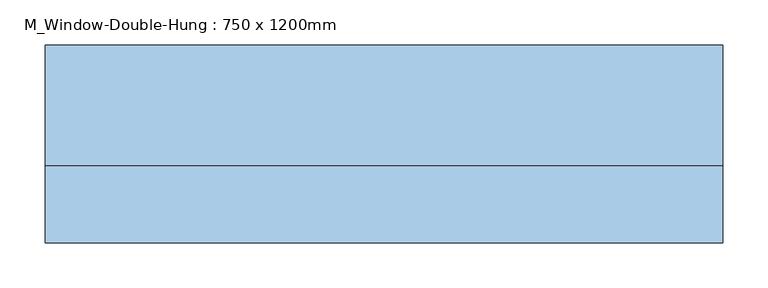
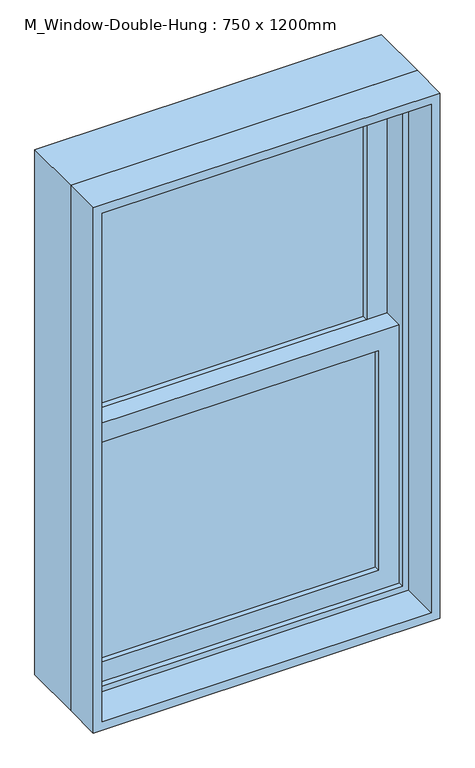
"""IFC4 building model written with IfcOpenShell, lengths in millimetres: window geometry, M_Window-Double-Hung : 750 x 1200mm."""

import ifcopenshell
import ifcopenshell.guid

model = None  # the IFC model being written
_history = None  # IfcOwnerHistory: only IFC2X3 demands one
_inside = {}  # id of a spatial element -> (the spatial element, [elements in it])
_under = {}  # id of a project, library or spatial element -> (it, [spatial elements below it])
_declared = {}  # id of a project -> (the project, [libraries it declares])
_typed = {}  # id of a type object -> (the type object, [elements of that type])
_made_of = {}  # id of a material, layer set ... -> (it, [elements and type objects made of it])


def new_model(schema):
    """Start an empty IFC model of exactly this schema.

    Asked for "IFC4X3", IfcOpenShell would pick the latest addendum, in which some entities
    have other attributes; the version numbers below select the first issue.
    IFC2X3 requires an IfcOwnerHistory on every rooted entity: one is made here for all.
    """
    global model, _history
    if schema == "IFC4X3":
        model = ifcopenshell.file(schema_version=(4, 3, 0, 0))
    else:
        model = ifcopenshell.file(schema=schema)
    _inside.clear()
    _under.clear()
    _declared.clear()
    _typed.clear()
    _made_of.clear()
    _history = None
    if model.schema == "IFC2X3":
        org = make("IfcOrganization", Name="unknown")
        user = make(
            "IfcPersonAndOrganization",
            ThePerson=make("IfcPerson", FamilyName="unknown"),
            TheOrganization=org,
        )
        app = make(
            "IfcApplication",
            ApplicationDeveloper=org,
            Version="unknown",
            ApplicationFullName="unknown",
            ApplicationIdentifier="unknown",
        )
        _history = make(
            "IfcOwnerHistory",
            OwningUser=user,
            OwningApplication=app,
            ChangeAction="ADDED",
            CreationDate=0,
        )
    return model


def make(cls, **values):
    """One entity of the class cls with the attributes given. An attribute that is None is left unset."""
    return model.create_entity(
        cls, **{name: value for name, value in values.items() if value is not None}
    )


def rooted(cls, **values):
    """An entity with a GlobalId (a new one), such as an element, a storey or a relation."""
    return make(cls, GlobalId=ifcopenshell.guid.new(), OwnerHistory=_history, **values)


def si_unit(unit_type, name, prefix=None):
    """IfcSIUnit, for example si_unit("LENGTHUNIT", "METRE", prefix="MILLI")."""
    return make("IfcSIUnit", UnitType=unit_type, Prefix=prefix, Name=name)


def assignment(units):
    """IfcUnitAssignment: the units of a project."""
    return None if units is None else make("IfcUnitAssignment", Units=units)


def point(xyz):
    """IfcCartesianPoint."""
    return None if xyz is None else make("IfcCartesianPoint", Coordinates=xyz)


def direction(xyz):
    """IfcDirection."""
    return None if xyz is None else make("IfcDirection", DirectionRatios=xyz)


def frame(location, z_axis=None, x_axis=None):
    """IfcAxis2Placement3D, a coordinate frame: its origin and axes. An axis left out is left unset."""
    return make(
        "IfcAxis2Placement3D",
        Location=point(location),
        Axis=direction(z_axis),
        RefDirection=direction(x_axis),
    )


def origin():
    """The frame at (0, 0, 0) with its axes left unset."""
    return frame((0.0, 0.0, 0.0))


def place(relative_to, where):
    """IfcLocalPlacement: puts the frame where relative to a parent placement (None: the world)."""
    return make(
        "IfcLocalPlacement", PlacementRelTo=relative_to, RelativePlacement=where
    )


def context(
    kind, dimensions, precision=None, world=None, true_north=None, identifier=None
):
    """IfcGeometricRepresentationContext, for example the 3D "Model" context."""
    return make(
        "IfcGeometricRepresentationContext",
        ContextIdentifier=identifier,
        ContextType=kind,
        CoordinateSpaceDimension=dimensions,
        Precision=precision,
        WorldCoordinateSystem=world,
        TrueNorth=true_north,
    )


def project(units=None, contexts=None):
    """IfcProject with its units and contexts."""
    return rooted(
        "IfcProject",
        Name="project",
        RepresentationContexts=contexts,
        UnitsInContext=assignment(units),
    )


def spatial(cls, under=None, at=None, **own):
    """A site, building, storey or space (cls), placed at a placement, below another one or the project."""
    s = rooted(cls, ObjectPlacement=at, **own)
    if under is not None:
        _under.setdefault(under.id(), (under, []))[1].append(s)
    return s


def polyline(points):
    """IfcPolyline through the points."""
    return make("IfcPolyline", Points=[point(p) for p in points])


def outline(outer, holes=None, kind="AREA"):
    """IfcArbitraryClosedProfileDef: a profile drawn as a closed curve; with holes, ...WithVoids."""
    if holes is None:
        return make("IfcArbitraryClosedProfileDef", ProfileType=kind, OuterCurve=outer)
    return make(
        "IfcArbitraryProfileDefWithVoids",
        ProfileType=kind,
        OuterCurve=outer,
        InnerCurves=holes,
    )


def extrude(swept, where, along, depth):
    """IfcExtrudedAreaSolid: the profile swept, set in the frame where, extruded along a direction by depth."""
    return make(
        "IfcExtrudedAreaSolid",
        SweptArea=swept,
        Position=where,
        ExtrudedDirection=direction(along),
        Depth=depth,
    )


def shape(context_of_items, identifier, shape_type, items):
    """IfcShapeRepresentation: the items that make up one representation, for example the "Body"."""
    return make(
        "IfcShapeRepresentation",
        ContextOfItems=context_of_items,
        RepresentationIdentifier=identifier,
        RepresentationType=shape_type,
        Items=items,
    )


def source(mapping_origin, context_of_items, identifier, shape_type, items):
    """IfcRepresentationMap: a shape defined once, which mapped items show again and again."""
    return make(
        "IfcRepresentationMap",
        MappingOrigin=mapping_origin,
        MappedRepresentation=shape(context_of_items, identifier, shape_type, items),
    )


def transform(
    local_origin,
    x_axis=None,
    y_axis=None,
    z_axis=None,
    scale=None,
    scale2=None,
    scale3=None,
    uniform=True,
):
    """IfcCartesianTransformationOperator3D, or its non-uniform kind. x_axis, y_axis, z_axis: its Axis1, 2, 3."""
    if uniform:
        return make(
            "IfcCartesianTransformationOperator3D",
            Axis1=direction(x_axis),
            Axis2=direction(y_axis),
            LocalOrigin=point(local_origin),
            Scale=scale,
            Axis3=direction(z_axis),
        )
    return make(
        "IfcCartesianTransformationOperator3DnonUniform",
        Axis1=direction(x_axis),
        Axis2=direction(y_axis),
        LocalOrigin=point(local_origin),
        Scale=scale,
        Axis3=direction(z_axis),
        Scale2=scale2,
        Scale3=scale3,
    )


def mapped(mapping_source, mapping_target):
    """IfcMappedItem: shows the shape of a source again, moved by a transform."""
    return make(
        "IfcMappedItem", MappingSource=mapping_source, MappingTarget=mapping_target
    )


def made_of(thing, what):
    """Note that an element or type object is made of a material, layer set ...; save() writes the relation."""
    if what is not None:
        _made_of.setdefault(what.id(), (what, []))[1].append(thing)
    return thing


def element(
    cls,
    number,
    at=None,
    inside=None,
    cuts=None,
    type_object=None,
    material=None,
    context=None,
    identifier="Body",
    shape_type=None,
    held_by="IfcProductDefinitionShape",
    body=None,
    shapes=None,
    **own,
):
    """One element of the class cls, such as IfcWall. Its Tag is "e" and its number.

    at: its placement. inside: the storey or other place that contains it. cuts: it is an
    opening in that element (IfcRelVoidsElement). A single representation is given by context,
    identifier, shape_type and body (its items); several are given by shapes. held_by: the class
    of the entity that holds the representations. save() writes the other relations.
    """
    e = rooted(cls, Tag="e%d" % number, ObjectPlacement=at, **own)
    if body is not None:
        shapes = [shape(context, identifier, shape_type, body)]
    if shapes is not None:
        e.Representation = make(held_by, Representations=shapes)
    if inside is not None:
        _inside.setdefault(inside.id(), (inside, []))[1].append(e)
    if cuts is not None:
        rooted(
            "IfcRelVoidsElement", RelatingBuildingElement=cuts, RelatedOpeningElement=e
        )
    if type_object is not None:
        _typed.setdefault(type_object.id(), (type_object, []))[1].append(e)
    return made_of(e, material)


def aggregate(whole, parts):
    """IfcRelAggregates: a whole, such as a stair, and the parts it consists of."""
    return rooted("IfcRelAggregates", RelatingObject=whole, RelatedObjects=parts)


def save(model, path):
    """Write the relations noted so far, then the file.

    IfcRelAggregates (storeys below a building ...), IfcRelContainedInSpatialStructure (elements
    in a storey), IfcRelDefinesByType, IfcRelAssociatesMaterial and IfcRelDeclares: one each for
    every whole, place, type object, material and project.
    """
    for whole, parts in _under.values():
        aggregate(whole, parts)
    for where, things in _inside.values():
        rooted(
            "IfcRelContainedInSpatialStructure",
            RelatedElements=things,
            RelatingStructure=where,
        )
    for kind, things in _typed.values():
        rooted("IfcRelDefinesByType", RelatedObjects=things, RelatingType=kind)
    for what, things in _made_of.values():
        rooted("IfcRelAssociatesMaterial", RelatedObjects=things, RelatingMaterial=what)
    for by, libraries in _declared.values():
        rooted("IfcRelDeclares", RelatingContext=by, RelatedDefinitions=libraries)
    model.write(path)


def m_window_double_hung_750_x_1200mm_41070976(model_context):
    return source(origin(), model_context, "Body", "SweptSolid", [
        extrude(outline(polyline([(298.8, 30.15), (298.8, 23.8), (-298.8, 23.8), (-298.8, 30.15), (298.8, 30.15)])), frame((0.0, 0.0, 990.6), z_axis=(0.0, 0.0, 1.0), x_axis=(1.0, 0.0, 0.0)), (0.0, 0.0, 1.0), 501.575),
        extrude(outline(polyline([(-298.8, 17.45), (298.8, 17.45), (298.8, 11.1), (-298.8, 11.1), (-298.8, 17.45)])), frame((0.0, 0.0, 990.6), z_axis=(0.0, 0.0, 1.0), x_axis=(1.0, 0.0, 0.0)), (0.0, 0.0, 1.0), 501.575),
        extrude(outline(polyline([(298.8, 74.6), (298.8, 68.25), (-298.8, 68.25), (-298.8, 74.6), (298.8, 74.6)])), frame((0.0, 0.0, 1536.625), z_axis=(0.0, 0.0, 1.0), x_axis=(1.0, 0.0, 0.0)), (0.0, 0.0, 1.0), 501.575),
        extrude(outline(polyline([(-298.8, 61.9), (298.8, 61.9), (298.8, 55.55), (-298.8, 55.55), (-298.8, 61.9)])), frame((0.0, 0.0, 1536.625), z_axis=(0.0, 0.0, 1.0), x_axis=(1.0, 0.0, 0.0)), (0.0, 0.0, 1.0), 501.575),
        extrude(outline(polyline([(1536.625, -343.25), (946.15, -343.25), (946.15, 343.25), (1536.625, 343.25), (1536.625, -343.25)]), holes=[polyline([(1492.175, 298.8), (990.6, 298.8), (990.6, -298.8), (1492.175, -298.8), (1492.175, 298.8)])]), frame((0.0, -1.6, 0.0), z_axis=(0.0, 1.0, 0.0), x_axis=(0.0, 0.0, 1.0)), (0.0, 0.0, 1.0), 44.45),
        extrude(outline(polyline([(2082.65, -343.25), (1492.175, -343.25), (1492.175, 343.25), (2082.65, 343.25), (2082.65, -343.25)]), holes=[polyline([(2038.2, 298.8), (1536.625, 298.8), (1536.625, -298.8), (2038.2, -298.8), (2038.2, 298.8)])]), frame((0.0, 42.85, 0.0), z_axis=(0.0, 1.0, 0.0), x_axis=(0.0, 0.0, 1.0)), (0.0, 0.0, 1.0), 44.45),
        extrude(outline(polyline([(2114.4, -375.0), (914.4, -375.0), (914.4, 375.0), (2114.4, 375.0), (2114.4, -375.0)]), holes=[polyline([(2082.65, 343.25), (946.15, 343.25), (946.15, -343.25), (2082.65, -343.25), (2082.65, 343.25)])]), frame((0.0, -14.3, 0.0), z_axis=(0.0, 1.0, 0.0), x_axis=(0.0, 0.0, 1.0)), (0.0, 0.0, 1.0), 133.35),
        extrude(outline(polyline([(2114.4, 375.0), (2114.4, -375.0), (914.4, -375.0), (914.4, 375.0), (2114.4, 375.0)]), holes=[polyline([(2095.35, 355.95), (933.45, 355.95), (933.45, -355.95), (2095.35, -355.95), (2095.35, 355.95)])]), frame((0.0, -100.0, 0.0), z_axis=(0.0, 1.0, 0.0), x_axis=(0.0, 0.0, 1.0)), (0.0, 0.0, 1.0), 85.7),
    ])


if __name__ == "__main__":
    model = new_model("IFC4")
    model_context = context("Model", 3, world=origin())
    ifc_project = project(units=[si_unit("LENGTHUNIT", "METRE", prefix="MILLI")], contexts=[model_context])
    site = spatial("IfcSite", under=ifc_project)
    building = spatial("IfcBuilding", under=site)
    placement = place(None, origin())
    m_window_double_hung_750_x_1200mm_shape = m_window_double_hung_750_x_1200mm_41070976(model_context)
    element("IfcWindow", 1, ObjectType="M_Window-Double-Hung : 750 x 1200mm", at=placement, inside=building, context=model_context, shape_type="MappedRepresentation", body=[
        mapped(m_window_double_hung_750_x_1200mm_shape, transform((0.0, 0.0, 0.0), x_axis=(1.0, 0.0, 0.0), y_axis=(0.0, 1.0, 0.0), z_axis=(0.0, 0.0, 1.0))),
    ])
    save(model, "model.ifc")

# Revit data of these elements
# Type "M_Window-Double-Hung : 750 x 1200mm"
#   Type Mark = "22"
#   Fire Rating = "0.5h"
#   Construction Type Id = "DG-DR"
#   Assembly Code = "B2020100"
#   Analytic Construction = "Double glazing - domestic"
#   Wall Thickness [instance default] = 150 mm
#   Window Inset [instance default] = 0 mm
#   Visual Light Transmittance = 0.81
#   Thermal Resistance (R) = 0.319569 (m²·K)/W
#   Solar Heat Gain Coefficient = 0.76
#   Muntin Width = 597.6 mm
#   Muntin Height = 501.575 mm
#   Interior Wall Closure [instance default] = 35.7 mm
#   Rough Width = 765 mm
#   Rough Height = 1215 mm
#   Frame Extension [instance default] = 31.75 mm
#   Exterior Wall Closure [instance default] = 12.7 mm
#   Extension Jamb [instance default] = 35.7 mm
#   Heat Transfer Coefficient (U) = 3.12929 W/(m²·K)
#   Height = 1200 mm
#   Width = 750 mm
#   Define Thermal Properties by = 1
#   Top Muntin Visibility = yes
#   Indicator Visibility [instance default] = yes
#   Extension Jamb Visibility [instance default] = yes
#   Interior Trim Visibility [instance default] = yes
#   Exterior Trim Visibility [instance default] = yes
#   Define Thermal Properties by = 1
#   Bottom Muntin Visibility = yes
#   Muntin Pattern = M_Muntin Pattern_2x2 : M_Muntin Pattern_2x2
#   Interior Trim Material = Wood - Stained
#   Interior Trim = M_Trim-Window-Interior-Flat : Picture Frame
#   Exterior Trim Material = Clad - White
#   Exterior Trim = M_Trim-Window-Exterior-Flat : with Sill
#   Glass Panel Material = Glass
#   Exterior Frame Material = Clad - White
#   Interior Frame Material = Wood - Stained
#   Wall Closure = (empty or 0)
# Element 1 (IfcWindow, "M_Window-Double-Hung : 750 x 1200mm")
#   Wall Thickness = 200 mm
#   Extension Jamb = 85.7 mm
#   Materials on its faces: "Wood - Stained", "Glass", "Clad - White"
# Materials
#   "Wood - Stained": class "Wood", colour RGB 224 178 126, transparency 0, Cost = 0
#   "Clad - White": class "Wood", colour RGB 242 242 238, transparency 0, Cost = 0
#   "Glass": class "Glass", colour RGB 0 128 192, transparency 0.9, Description = "Soda Lime Glass", Cost = 0
